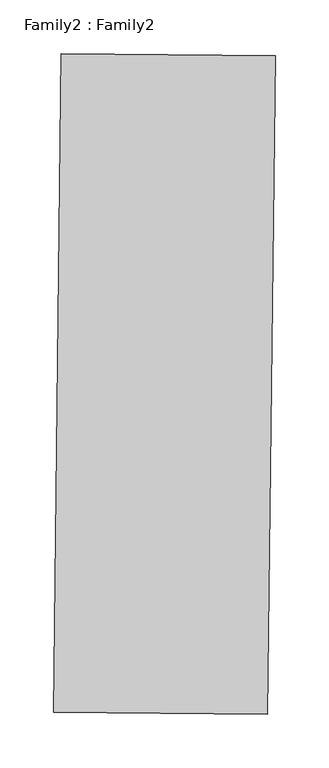
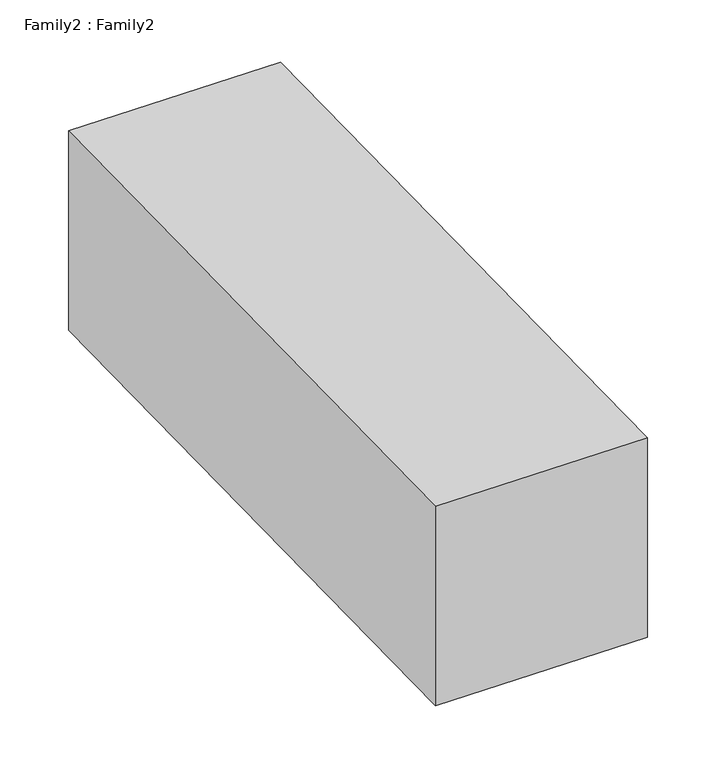
"""IFC4 building model written with IfcOpenShell, lengths in millimetres: proxy geometry, Family2 : Family2."""

from ifc_helpers import new_model, si_unit, origin, place, context, project, spatial, faceted_brep, source, transform, mapped, element, save


def family2_family2_49637704(model_context):
    return source(origin(), model_context, "Body", "Brep", [
        faceted_brep([(-3947.1236849, -6381.446434, 1.0945136), (-3947.1236849, -6381.446434, 201.0945136), (-3939.7191096, -5766.1536886, 202.060409), (-3939.7191096, -5766.1536886, 2.060409), (-3747.1324949, -6383.3236466, 201.0945136), (-3739.7279196, -5768.0309013, 202.060409), (-3747.1324949, -6383.3236466, 1.0945136), (-3739.7279196, -5768.0309013, 2.060409)], [[[0, 1, 2, 3]], [[1, 4, 5, 2]], [[4, 6, 7, 5]], [[6, 0, 3, 7]], [[3, 2, 5, 7]], [[0, 6, 4, 1]]]),
    ])


if __name__ == "__main__":
    model = new_model("IFC4")
    model_context = context("Model", 3, world=origin())
    ifc_project = project(units=[si_unit("LENGTHUNIT", "METRE", prefix="MILLI")], contexts=[model_context])
    site = spatial("IfcSite", under=ifc_project)
    building = spatial("IfcBuilding", under=site)
    placement = place(None, origin())
    family2_family2_shape = family2_family2_49637704(model_context)
    element("IfcBuildingElementProxy", 1, Name="Family2 : Family2", ObjectType="Family2 : Family2", at=placement, inside=building, context=model_context, shape_type="MappedRepresentation", body=[
        mapped(family2_family2_shape, transform((0.0, 0.0, 0.0), x_axis=(1.0, 0.0, 0.0), y_axis=(0.0, 1.0, 0.0), z_axis=(0.0, 0.0, 1.0))),
    ])
    save(model, "model.ifc")

# Revit data of these elements
# Type "Family2 : Family2"
#   Default Elevation = 0
